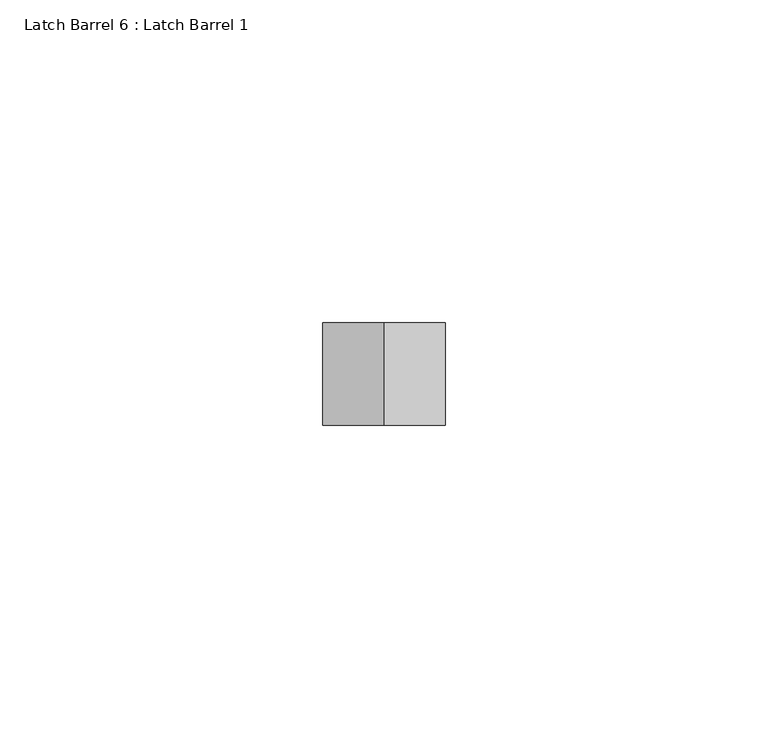
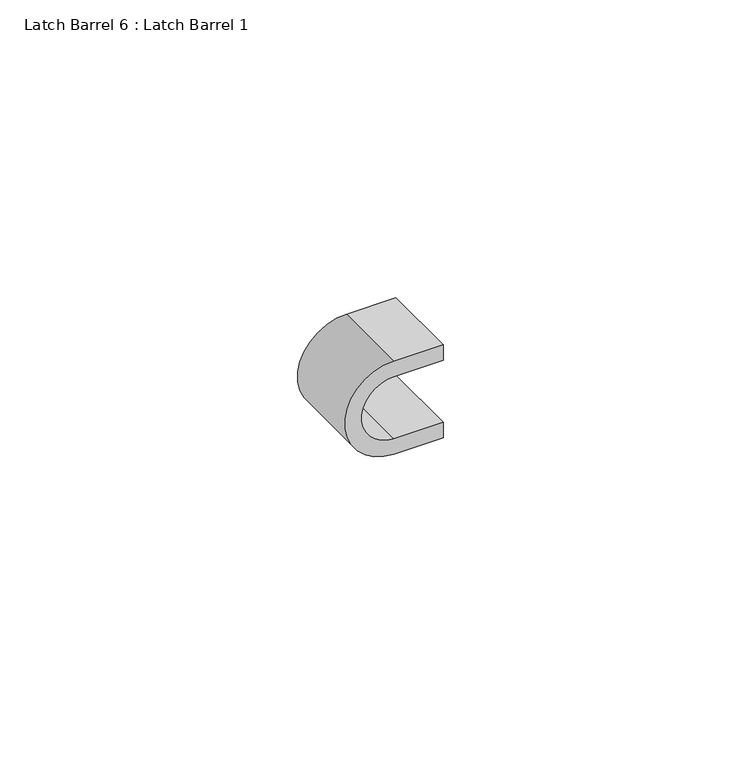
"""IFC4 building model written with IfcOpenShell, lengths in millimetres: proxy geometry, Latch Barrel 6 : Latch Barrel 1."""

from ifc_helpers import new_model, si_unit, point, frame, frame_2d, origin, place, context, project, spatial, polyline, circle_curve, trimmed, segment, composite_curve, outline, extrude, source, transform, mapped, element, save


def latch_barrel_6_latch_barrel_1_3a8c0b8a(model_context):
    return source(origin(), model_context, "Body", "SweptSolid", [
        extrude(outline(composite_curve([segment(trimmed(circle_curve(frame_2d((1066.8, 587312.7185739)), 6.35), [point((1060.45, 587312.7185739))], [point((1073.15, 587312.7185739))], True, "CARTESIAN"), True, "CONTINUOUS"), segment(polyline([(1073.15, 587312.7185739), (1073.15, 587322.2435739), (1076.325, 587322.2435739), (1076.325, 587312.7185739)]), True, "CONTINUOUS"), segment(trimmed(circle_curve(frame_2d((1066.8, 587312.7185739)), 9.525), [point((1076.325, 587312.7185739))], [point((1057.275, 587312.7185739))], False, "CARTESIAN"), True, "CONTINUOUS"), segment(polyline([(1057.275, 587312.7185739), (1057.275, 587322.2435739), (1060.45, 587322.2435739), (1060.45, 587312.7185739)]), True, "CONTINUOUS")], self_intersect=False)), frame((0.0, -535230.1413841, 0.0), z_axis=(0.0, 1.0, 0.0), x_axis=(0.0, 0.0, 1.0)), (0.0, 0.0, 1.0), 15.875),
    ])


if __name__ == "__main__":
    model = new_model("IFC4")
    model_context = context("Model", 3, world=origin())
    ifc_project = project(units=[si_unit("LENGTHUNIT", "METRE", prefix="MILLI")], contexts=[model_context])
    site = spatial("IfcSite", under=ifc_project)
    building = spatial("IfcBuilding", under=site)
    placement = place(None, origin())
    latch_barrel_6_latch_barrel_1_shape = latch_barrel_6_latch_barrel_1_3a8c0b8a(model_context)
    element("IfcBuildingElementProxy", 1, Name="Latch Barrel 6 : Latch Barrel 1", ObjectType="Latch Barrel 6 : Latch Barrel 1", at=placement, inside=building, context=model_context, shape_type="MappedRepresentation", body=[
        mapped(latch_barrel_6_latch_barrel_1_shape, transform((0.0, 0.0, 0.0), x_axis=(1.0, 0.0, 0.0), y_axis=(0.0, 1.0, 0.0), z_axis=(0.0, 0.0, 1.0))),
    ])
    save(model, "model.ifc")

# Revit data of these elements
# Element 1 (IfcBuildingElementProxy, "Latch Barrel 6 : Latch Barrel 1")
#   Materials on its faces: "GALV. GATE LATCH"
# Materials
#   "GALV. GATE LATCH": class "Metal", colour RGB 189 187 185, transparency 0, Description = "Carbon steel", Cost = 0
